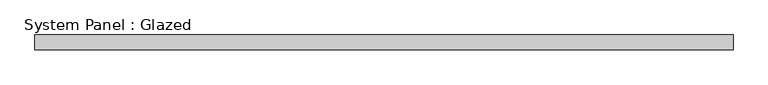
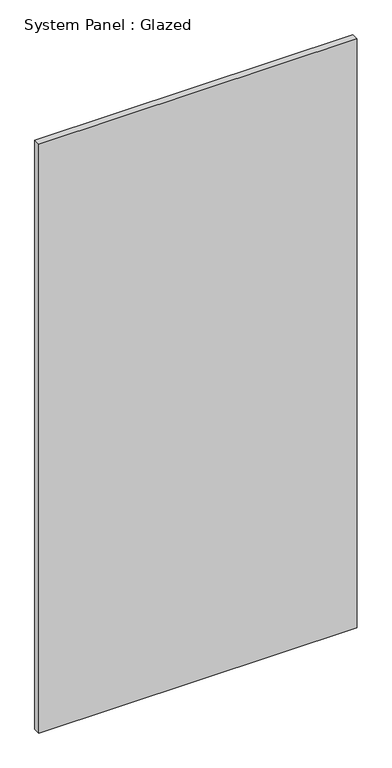
"""IFC4 building model written with IfcOpenShell, lengths in millimetres: plate geometry, System Panel : Glazed."""

from ifc_helpers import new_model, si_unit, origin, origin_with_axes, place, context, project, spatial, polyline, outline, extrude, source, transform, mapped, element, save


def system_panel_glazed_cc393cf4(model_context):
    return source(origin(), model_context, "Body", "SweptSolid", [
        extrude(outline(polyline([(599.0166667, 19.05), (-599.0166667, 19.05), (-599.0166667, 44.45), (599.0166667, 44.45), (599.0166667, 19.05)])), origin_with_axes(), (0.0, 0.0, 1.0), 2343.15),
    ])


if __name__ == "__main__":
    model = new_model("IFC4")
    model_context = context("Model", 3, world=origin())
    ifc_project = project(units=[si_unit("LENGTHUNIT", "METRE", prefix="MILLI")], contexts=[model_context])
    site = spatial("IfcSite", under=ifc_project)
    building = spatial("IfcBuilding", under=site)
    placement = place(None, origin())
    system_panel_glazed_shape = system_panel_glazed_cc393cf4(model_context)
    element("IfcPlate", 1, ObjectType="System Panel : Glazed", at=placement, inside=building, context=model_context, shape_type="MappedRepresentation", body=[
        mapped(system_panel_glazed_shape, transform((0.0, 0.0, 0.0), x_axis=(1.0, 0.0, 0.0), y_axis=(0.0, 1.0, 0.0), z_axis=(0.0, 0.0, 1.0))),
    ])
    save(model, "model.ifc")

# Revit data of these elements
# Element 1 (IfcPlate, "System Panel : Glazed")
#   Materials on its faces: "Glass"
# Materials
#   "Glass": class "Glass", colour RGB 218 227 224, transparency 0.85, Description = "Soda Lime Glass", Cost = 0
